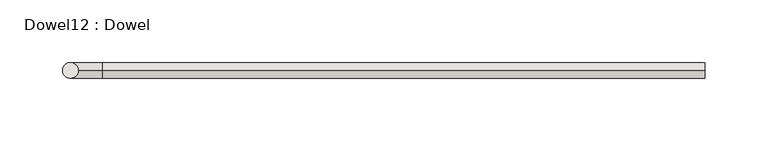
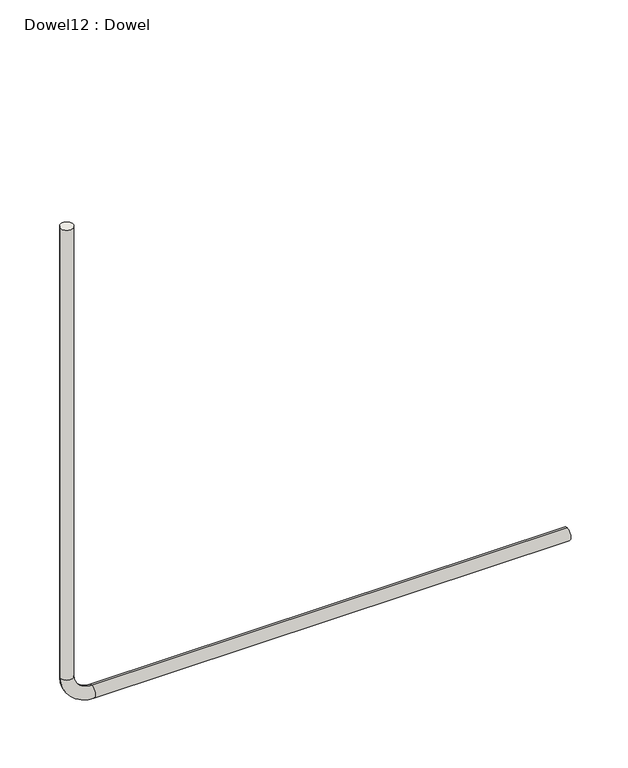
"""IFC4 building model written with IfcOpenShell, lengths in millimetres: wall geometry, Dowel12 : Dowel."""

from ifc_helpers import new_model, si_unit, point, frame, origin, place, context, project, spatial, circle_curve, ellipse_curve, trimmed, source, transform, mapped, element, save
from ifc_brep_helpers import plane_surface, cylinder_surface, revolved_surface, advanced_brep


def dowel12_dowel_70360233(model_context):
    return source(origin(), model_context, "Body", "AdvancedBrep", [
        advanced_brep(
        [(375079.9410859, 446.88125, 2616.3420731), (375092.6410859, 446.88125, 2616.3420731), (375079.9410859, 446.88125, 2133.7420731), (375092.6410859, 446.88125, 2133.7420731), (375111.6910859, 446.88125, 2114.6920731), (375111.6910859, 446.88125, 2101.9920731), (375594.2910859, 446.88125, 2101.9920731), (375594.2910859, 446.88125, 2114.6920731)],
        [
            (0, 1, circle_curve(frame((375086.2910859, 446.88125, 2616.3420731), z_axis=(0.0, 0.0, 1.0), x_axis=(1.0, 0.0, 0.0)), 6.35)),
            (1, 0, circle_curve(frame((375086.2910859, 446.88125, 2616.3420731), z_axis=(0.0, 0.0, 1.0), x_axis=(1.0, 0.0, 0.0)), 6.35)),
            (0, 2),
            (2, 3, circle_curve(frame((375086.2910859, 446.88125, 2133.7420731), z_axis=(0.0, 0.0, 1.0), x_axis=(1.0, 0.0, 0.0)), 6.35)),
            (3, 1),
            (3, 2, circle_curve(frame((375086.2910859, 446.88125, 2133.7420731), z_axis=(0.0, 0.0, 1.0), x_axis=(1.0, 0.0, 0.0)), 6.35)),
            (4, 3, circle_curve(frame((375111.6910859, 446.88125, 2133.7420731), z_axis=(0.0, 1.0, 0.0), x_axis=(-1.0, 0.0, 0.0)), 19.05)),
            (2, 5, circle_curve(frame((375111.6910859, 446.88125, 2133.7420731), z_axis=(0.0, -1.0, 0.0), x_axis=(-1.0, 0.0, 0.0)), 31.75)),
            (5, 4, circle_curve(frame((375111.6910859, 446.88125, 2108.3420731), z_axis=(-1.0, 0.0, 0.0), x_axis=(0.0, 0.0, 1.0)), 6.35)),
            (4, 5, circle_curve(frame((375111.6910859, 446.88125, 2108.3420731), z_axis=(-1.0, 0.0, 0.0), x_axis=(0.0, 0.0, 1.0)), 6.35)),
            (6, 7, circle_curve(frame((375594.2910859, 446.88125, 2108.3420731), z_axis=(1.0, 0.0, 0.0), x_axis=(0.0, 0.0, 1.0)), 6.35)),
            (7, 6, circle_curve(frame((375594.2910859, 446.88125, 2108.3420731), z_axis=(1.0, 0.0, 0.0), x_axis=(0.0, 0.0, 1.0)), 6.35)),
            (5, 6),
            (7, 4),
        ],
        [
            plane_surface(frame((375086.2910859, 446.88125, 2616.3420731), z_axis=(0.0, 0.0, 1.0), x_axis=(0.0, -1.0, 0.0))),
            cylinder_surface(frame((375086.2910859, 446.88125, 2616.3420731), z_axis=(0.0, 0.0, 1.0), x_axis=(1.0, 0.0, 0.0)), 6.35),
            revolved_surface(trimmed(ellipse_curve(frame((375086.2910859, 446.88125, 2133.7420731), z_axis=(0.0, 0.0, 1.0), x_axis=(1.0, 0.0, 0.0)), 6.35, 6.35), [point((375079.9410859, 446.88125, 2133.7420731))], [point((375092.6410859, 446.88125, 2133.7420731))], True, "CARTESIAN"), (375111.6910859, 446.88125, 2133.7420731), (0.0, -1.0, 0.0)),
            revolved_surface(trimmed(ellipse_curve(frame((375086.2910859, 446.88125, 2133.7420731), z_axis=(0.0, 0.0, 1.0), x_axis=(1.0, 0.0, 0.0)), 6.35, 6.35), [point((375092.6410859, 446.88125, 2133.7420731))], [point((375079.9410859, 446.88125, 2133.7420731))], True, "CARTESIAN"), (375111.6910859, 446.88125, 2133.7420731), (0.0, -1.0, 0.0)),
            plane_surface(frame((375594.2910859, 446.88125, 2108.3420731), z_axis=(1.0, 0.0, 0.0), x_axis=(0.0, -1.0, 0.0))),
            cylinder_surface(frame((375111.6910859, 446.88125, 2108.3420731), z_axis=(-1.0, 0.0, 0.0), x_axis=(0.0, 0.0, 1.0)), 6.35),
        ],
        [
            (0, [[1, 2]]),
            (1, [[-1, 3, 4, 5]]),
            (1, [[-2, -5, 6, -3]]),
            (2, [[7, -4, 8, 9]]),
            (3, [[-8, -6, -7, 10]]),
            (4, [[11, 12]]),
            (5, [[-9, 13, -12, 14]]),
            (5, [[-10, -14, -11, -13]]),
        ],
    ),
    ])


if __name__ == "__main__":
    model = new_model("IFC4")
    model_context = context("Model", 3, world=origin())
    ifc_project = project(units=[si_unit("LENGTHUNIT", "METRE", prefix="MILLI")], contexts=[model_context])
    site = spatial("IfcSite", under=ifc_project)
    building = spatial("IfcBuilding", under=site)
    placement = place(None, origin())
    dowel12_dowel_shape = dowel12_dowel_70360233(model_context)
    element("IfcWall", 1, ObjectType="Dowel12 : Dowel", at=placement, inside=building, context=model_context, shape_type="MappedRepresentation", body=[
        mapped(dowel12_dowel_shape, transform((0.0, 0.0, 0.0), x_axis=(1.0, 0.0, 0.0), y_axis=(0.0, 1.0, 0.0), z_axis=(0.0, 0.0, 1.0))),
    ])
    save(model, "model.ifc")

# Revit data of these elements
# Element 1 (IfcWall, "Dowel12 : Dowel")
#   Materials on its faces: "#4 J's @ 24\" O.C. - GROUTED IN PRECAST KEYS AND CORES"
# Materials
#   "#4 J's @ 24\" O.C. - GROUTED IN PRECAST KEYS AND CORES": class "Generic", colour RGB 255 255 255, transparency 0, Cost = 0
